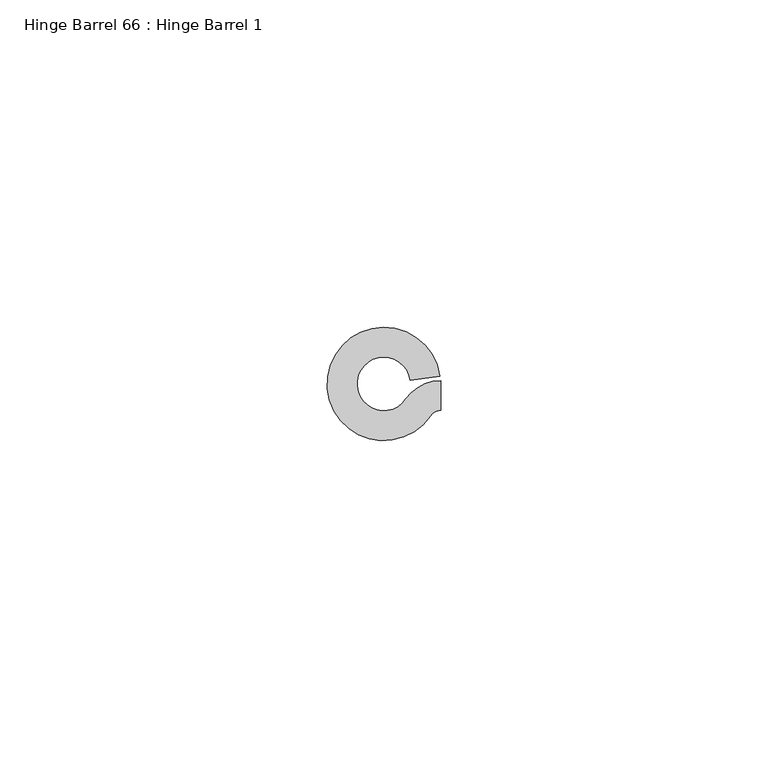
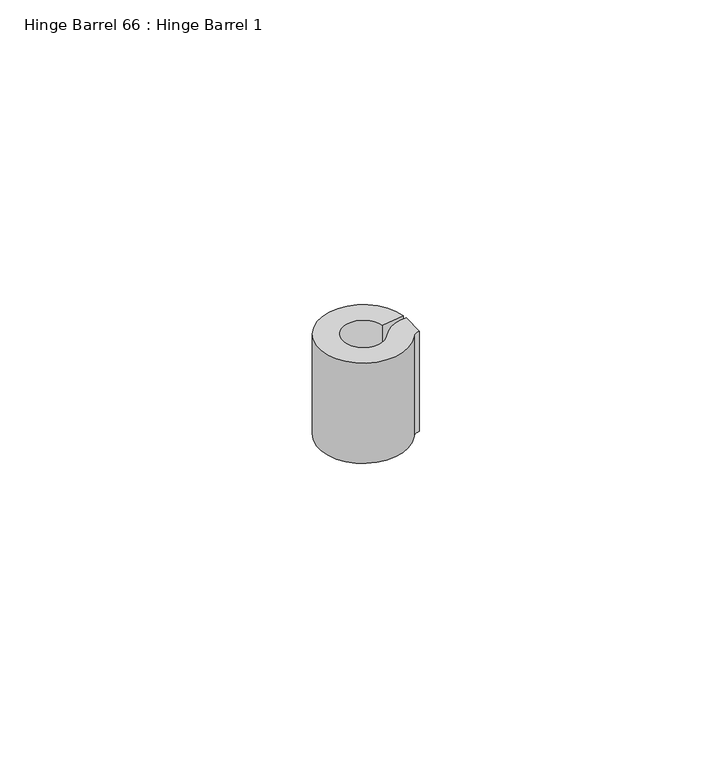
"""IFC4 building model written with IfcOpenShell, lengths in millimetres: proxy geometry, Hinge Barrel 66 : Hinge Barrel 1."""

from ifc_helpers import new_model, si_unit, point, frame, frame_2d, origin, place, context, project, spatial, polyline, circle_curve, trimmed, segment, composite_curve, outline, extrude, source, transform, mapped, element, save


def hinge_barrel_66_hinge_barrel_1_4b45ecc4(model_context):
    return source(origin(), model_context, "Body", "SweptSolid", [
        extrude(outline(composite_curve([segment(trimmed(circle_curve(frame_2d((587327.8245257, -536316.2443067)), 6.4044851), [point((587322.5194669, -536312.6563017))], [point((587327.8245257, -536309.8398216))], False, "CARTESIAN"), True, "CONTINUOUS"), segment(polyline([(587327.8245257, -536309.8398216), (587327.8245257, -536314.4038841)]), True, "CONTINUOUS"), segment(trimmed(circle_curve(frame_2d((587327.8245257, -536316.2443067)), 1.8404226), [point((587327.8245257, -536314.4038841))], [point((587326.3000393, -536315.2132409))], True, "CARTESIAN"), True, "CONTINUOUS"), segment(trimmed(circle_curve(frame_2d((587319.1320739, -536310.3652841)), 8.6534625), [point((587326.3000393, -536315.2132409))], [point((587327.7022899, -536309.1678654))], False, "CARTESIAN"), True, "CONTINUOUS"), segment(polyline([(587327.7022899, -536309.1678654), (587323.1821338, -536309.7994153)]), True, "CONTINUOUS"), segment(trimmed(circle_curve(frame_2d((587319.1320739, -536310.3652841)), 4.0894), [point((587323.1821338, -536309.7994153))], [point((587322.5194669, -536312.6563017))], True, "CARTESIAN"), True, "CONTINUOUS")], self_intersect=False)), frame((0.0, 0.0, 2063.75), z_axis=(0.0, 0.0, 1.0), x_axis=(1.0, 0.0, 0.0)), (0.0, 0.0, 1.0), 20.8359375),
    ])


if __name__ == "__main__":
    model = new_model("IFC4")
    model_context = context("Model", 3, world=origin())
    ifc_project = project(units=[si_unit("LENGTHUNIT", "METRE", prefix="MILLI")], contexts=[model_context])
    site = spatial("IfcSite", under=ifc_project)
    building = spatial("IfcBuilding", under=site)
    placement = place(None, origin())
    hinge_barrel_66_hinge_barrel_1_shape = hinge_barrel_66_hinge_barrel_1_4b45ecc4(model_context)
    element("IfcBuildingElementProxy", 1, Name="Hinge Barrel 66 : Hinge Barrel 1", ObjectType="Hinge Barrel 66 : Hinge Barrel 1", at=placement, inside=building, context=model_context, shape_type="MappedRepresentation", body=[
        mapped(hinge_barrel_66_hinge_barrel_1_shape, transform((0.0, 0.0, 0.0), x_axis=(1.0, 0.0, 0.0), y_axis=(0.0, 1.0, 0.0), z_axis=(0.0, 0.0, 1.0))),
    ])
    save(model, "model.ifc")

# Revit data of these elements
# Element 1 (IfcBuildingElementProxy, "Hinge Barrel 66 : Hinge Barrel 1")
#   Materials on its faces: "6\"X6\" WELD-ON STL BUTT HINGE"
# Materials
#   "6\"X6\" WELD-ON STL BUTT HINGE": class "Metal", colour RGB 189 187 185, transparency 0, Description = "Carbon steel", Cost = 0
